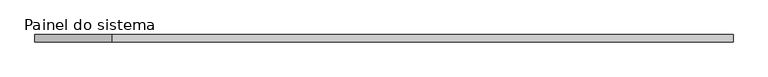
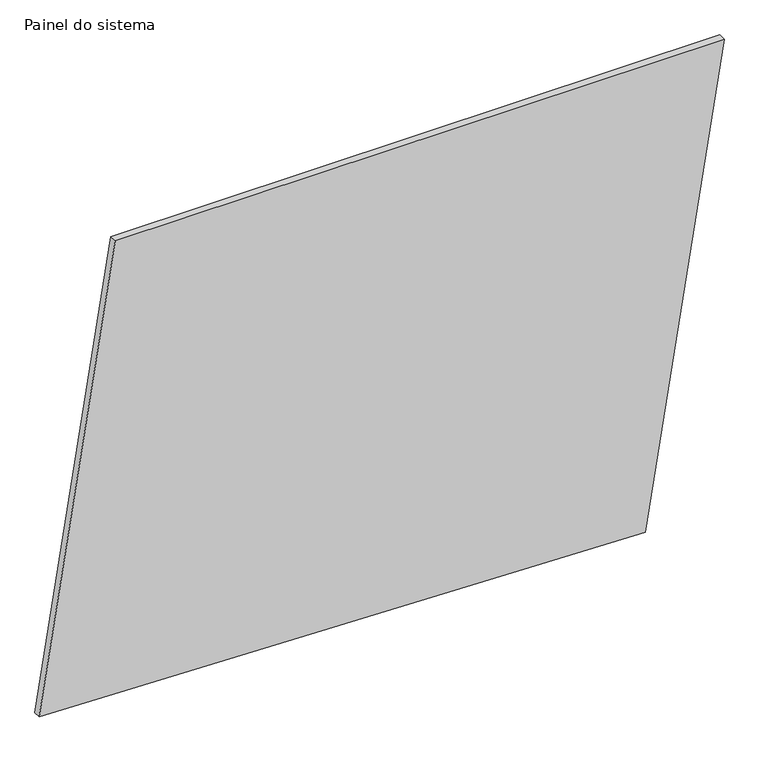
"""IFC4 building model written with IfcOpenShell, lengths in millimetres: plate geometry, Painel do sistema : Envidraçado."""

import ifcopenshell
import ifcopenshell.guid

model = None  # the IFC model being written
_history = None  # IfcOwnerHistory: only IFC2X3 demands one
_inside = {}  # id of a spatial element -> (the spatial element, [elements in it])
_under = {}  # id of a project, library or spatial element -> (it, [spatial elements below it])
_declared = {}  # id of a project -> (the project, [libraries it declares])
_typed = {}  # id of a type object -> (the type object, [elements of that type])
_made_of = {}  # id of a material, layer set ... -> (it, [elements and type objects made of it])


def new_model(schema):
    """Start an empty IFC model of exactly this schema.

    Asked for "IFC4X3", IfcOpenShell would pick the latest addendum, in which some entities
    have other attributes; the version numbers below select the first issue.
    IFC2X3 requires an IfcOwnerHistory on every rooted entity: one is made here for all.
    """
    global model, _history
    if schema == "IFC4X3":
        model = ifcopenshell.file(schema_version=(4, 3, 0, 0))
    else:
        model = ifcopenshell.file(schema=schema)
    _inside.clear()
    _under.clear()
    _declared.clear()
    _typed.clear()
    _made_of.clear()
    _history = None
    if model.schema == "IFC2X3":
        org = make("IfcOrganization", Name="unknown")
        user = make(
            "IfcPersonAndOrganization",
            ThePerson=make("IfcPerson", FamilyName="unknown"),
            TheOrganization=org,
        )
        app = make(
            "IfcApplication",
            ApplicationDeveloper=org,
            Version="unknown",
            ApplicationFullName="unknown",
            ApplicationIdentifier="unknown",
        )
        _history = make(
            "IfcOwnerHistory",
            OwningUser=user,
            OwningApplication=app,
            ChangeAction="ADDED",
            CreationDate=0,
        )
    return model


def make(cls, **values):
    """One entity of the class cls with the attributes given. An attribute that is None is left unset."""
    return model.create_entity(
        cls, **{name: value for name, value in values.items() if value is not None}
    )


def rooted(cls, **values):
    """An entity with a GlobalId (a new one), such as an element, a storey or a relation."""
    return make(cls, GlobalId=ifcopenshell.guid.new(), OwnerHistory=_history, **values)


def si_unit(unit_type, name, prefix=None):
    """IfcSIUnit, for example si_unit("LENGTHUNIT", "METRE", prefix="MILLI")."""
    return make("IfcSIUnit", UnitType=unit_type, Prefix=prefix, Name=name)


def assignment(units):
    """IfcUnitAssignment: the units of a project."""
    return None if units is None else make("IfcUnitAssignment", Units=units)


def point(xyz):
    """IfcCartesianPoint."""
    return None if xyz is None else make("IfcCartesianPoint", Coordinates=xyz)


def direction(xyz):
    """IfcDirection."""
    return None if xyz is None else make("IfcDirection", DirectionRatios=xyz)


def frame(location, z_axis=None, x_axis=None):
    """IfcAxis2Placement3D, a coordinate frame: its origin and axes. An axis left out is left unset."""
    return make(
        "IfcAxis2Placement3D",
        Location=point(location),
        Axis=direction(z_axis),
        RefDirection=direction(x_axis),
    )


def origin():
    """The frame at (0, 0, 0) with its axes left unset."""
    return frame((0.0, 0.0, 0.0))


def place(relative_to, where):
    """IfcLocalPlacement: puts the frame where relative to a parent placement (None: the world)."""
    return make(
        "IfcLocalPlacement", PlacementRelTo=relative_to, RelativePlacement=where
    )


def context(
    kind, dimensions, precision=None, world=None, true_north=None, identifier=None
):
    """IfcGeometricRepresentationContext, for example the 3D "Model" context."""
    return make(
        "IfcGeometricRepresentationContext",
        ContextIdentifier=identifier,
        ContextType=kind,
        CoordinateSpaceDimension=dimensions,
        Precision=precision,
        WorldCoordinateSystem=world,
        TrueNorth=true_north,
    )


def project(units=None, contexts=None):
    """IfcProject with its units and contexts."""
    return rooted(
        "IfcProject",
        Name="project",
        RepresentationContexts=contexts,
        UnitsInContext=assignment(units),
    )


def spatial(cls, under=None, at=None, **own):
    """A site, building, storey or space (cls), placed at a placement, below another one or the project."""
    s = rooted(cls, ObjectPlacement=at, **own)
    if under is not None:
        _under.setdefault(under.id(), (under, []))[1].append(s)
    return s


def polyline(points):
    """IfcPolyline through the points."""
    return make("IfcPolyline", Points=[point(p) for p in points])


def outline(outer, holes=None, kind="AREA"):
    """IfcArbitraryClosedProfileDef: a profile drawn as a closed curve; with holes, ...WithVoids."""
    if holes is None:
        return make("IfcArbitraryClosedProfileDef", ProfileType=kind, OuterCurve=outer)
    return make(
        "IfcArbitraryProfileDefWithVoids",
        ProfileType=kind,
        OuterCurve=outer,
        InnerCurves=holes,
    )


def extrude(swept, where, along, depth):
    """IfcExtrudedAreaSolid: the profile swept, set in the frame where, extruded along a direction by depth."""
    return make(
        "IfcExtrudedAreaSolid",
        SweptArea=swept,
        Position=where,
        ExtrudedDirection=direction(along),
        Depth=depth,
    )


def shape(context_of_items, identifier, shape_type, items):
    """IfcShapeRepresentation: the items that make up one representation, for example the "Body"."""
    return make(
        "IfcShapeRepresentation",
        ContextOfItems=context_of_items,
        RepresentationIdentifier=identifier,
        RepresentationType=shape_type,
        Items=items,
    )


def source(mapping_origin, context_of_items, identifier, shape_type, items):
    """IfcRepresentationMap: a shape defined once, which mapped items show again and again."""
    return make(
        "IfcRepresentationMap",
        MappingOrigin=mapping_origin,
        MappedRepresentation=shape(context_of_items, identifier, shape_type, items),
    )


def transform(
    local_origin,
    x_axis=None,
    y_axis=None,
    z_axis=None,
    scale=None,
    scale2=None,
    scale3=None,
    uniform=True,
):
    """IfcCartesianTransformationOperator3D, or its non-uniform kind. x_axis, y_axis, z_axis: its Axis1, 2, 3."""
    if uniform:
        return make(
            "IfcCartesianTransformationOperator3D",
            Axis1=direction(x_axis),
            Axis2=direction(y_axis),
            LocalOrigin=point(local_origin),
            Scale=scale,
            Axis3=direction(z_axis),
        )
    return make(
        "IfcCartesianTransformationOperator3DnonUniform",
        Axis1=direction(x_axis),
        Axis2=direction(y_axis),
        LocalOrigin=point(local_origin),
        Scale=scale,
        Axis3=direction(z_axis),
        Scale2=scale2,
        Scale3=scale3,
    )


def mapped(mapping_source, mapping_target):
    """IfcMappedItem: shows the shape of a source again, moved by a transform."""
    return make(
        "IfcMappedItem", MappingSource=mapping_source, MappingTarget=mapping_target
    )


def made_of(thing, what):
    """Note that an element or type object is made of a material, layer set ...; save() writes the relation."""
    if what is not None:
        _made_of.setdefault(what.id(), (what, []))[1].append(thing)
    return thing


def element(
    cls,
    number,
    at=None,
    inside=None,
    cuts=None,
    type_object=None,
    material=None,
    context=None,
    identifier="Body",
    shape_type=None,
    held_by="IfcProductDefinitionShape",
    body=None,
    shapes=None,
    **own,
):
    """One element of the class cls, such as IfcWall. Its Tag is "e" and its number.

    at: its placement. inside: the storey or other place that contains it. cuts: it is an
    opening in that element (IfcRelVoidsElement). A single representation is given by context,
    identifier, shape_type and body (its items); several are given by shapes. held_by: the class
    of the entity that holds the representations. save() writes the other relations.
    """
    e = rooted(cls, Tag="e%d" % number, ObjectPlacement=at, **own)
    if body is not None:
        shapes = [shape(context, identifier, shape_type, body)]
    if shapes is not None:
        e.Representation = make(held_by, Representations=shapes)
    if inside is not None:
        _inside.setdefault(inside.id(), (inside, []))[1].append(e)
    if cuts is not None:
        rooted(
            "IfcRelVoidsElement", RelatingBuildingElement=cuts, RelatedOpeningElement=e
        )
    if type_object is not None:
        _typed.setdefault(type_object.id(), (type_object, []))[1].append(e)
    return made_of(e, material)


def aggregate(whole, parts):
    """IfcRelAggregates: a whole, such as a stair, and the parts it consists of."""
    return rooted("IfcRelAggregates", RelatingObject=whole, RelatedObjects=parts)


def save(model, path):
    """Write the relations noted so far, then the file.

    IfcRelAggregates (storeys below a building ...), IfcRelContainedInSpatialStructure (elements
    in a storey), IfcRelDefinesByType, IfcRelAssociatesMaterial and IfcRelDeclares: one each for
    every whole, place, type object, material and project.
    """
    for whole, parts in _under.values():
        aggregate(whole, parts)
    for where, things in _inside.values():
        rooted(
            "IfcRelContainedInSpatialStructure",
            RelatedElements=things,
            RelatingStructure=where,
        )
    for kind, things in _typed.values():
        rooted("IfcRelDefinesByType", RelatedObjects=things, RelatingType=kind)
    for what, things in _made_of.values():
        rooted("IfcRelAssociatesMaterial", RelatedObjects=things, RelatingMaterial=what)
    for by, libraries in _declared.values():
        rooted("IfcRelDeclares", RelatingContext=by, RelatedDefinitions=libraries)
    model.write(path)


def painel_do_sistema_7608f2ac(model_context):
    return source(origin(), model_context, "Body", "SweptSolid", [
        extrude(outline(polyline([(58.8334996, -1174.3666445), (0.0, 904.1711245), (1693.8529641, 1174.3666445), (1693.8529641, -913.5559698), (58.8334996, -1174.3666445)])), frame((0.0, 24.5, 0.0), z_axis=(0.0, 1.0, 0.0), x_axis=(0.0, 0.0, 1.0)), (0.0, 0.0, 1.0), 25.0),
    ])


if __name__ == "__main__":
    model = new_model("IFC4")
    model_context = context("Model", 3, world=origin())
    ifc_project = project(units=[si_unit("LENGTHUNIT", "METRE", prefix="MILLI")], contexts=[model_context])
    site = spatial("IfcSite", under=ifc_project)
    building = spatial("IfcBuilding", under=site)
    placement = place(None, origin())
    painel_do_sistema_shape = painel_do_sistema_7608f2ac(model_context)
    element("IfcPlate", 1, ObjectType="Painel do sistema : Envidraçado", at=placement, inside=building, context=model_context, shape_type="MappedRepresentation", body=[
        mapped(painel_do_sistema_shape, transform((0.0, 0.0, 0.0), x_axis=(1.0, 0.0, 0.0), y_axis=(0.0, 1.0, 0.0), z_axis=(0.0, 0.0, 1.0))),
    ])
    save(model, "model.ifc")

# Revit data of these elements
# Type "Painel do sistema : Envidraçado"
#   Construction Type Id = "GSP4R"
#   Analytic Construction = "Vidraça única Pilkington 1/8 pol"
#   Visual Light Transmittance = 0.9
#   Solar Heat Gain Coefficient = 0.86
#   Heat Transfer Coefficient (U) = 6.7069 W/(m²·K)
# Element 1 (IfcPlate, "Painel do sistema : Envidraçado")
#   Materials on its faces: "Vidro"
# Materials
#   "Vidro": class "Vidro", colour RGB 0 128 192, transparency 0.9, Description = "Vidro de sílica", Cost = 0
